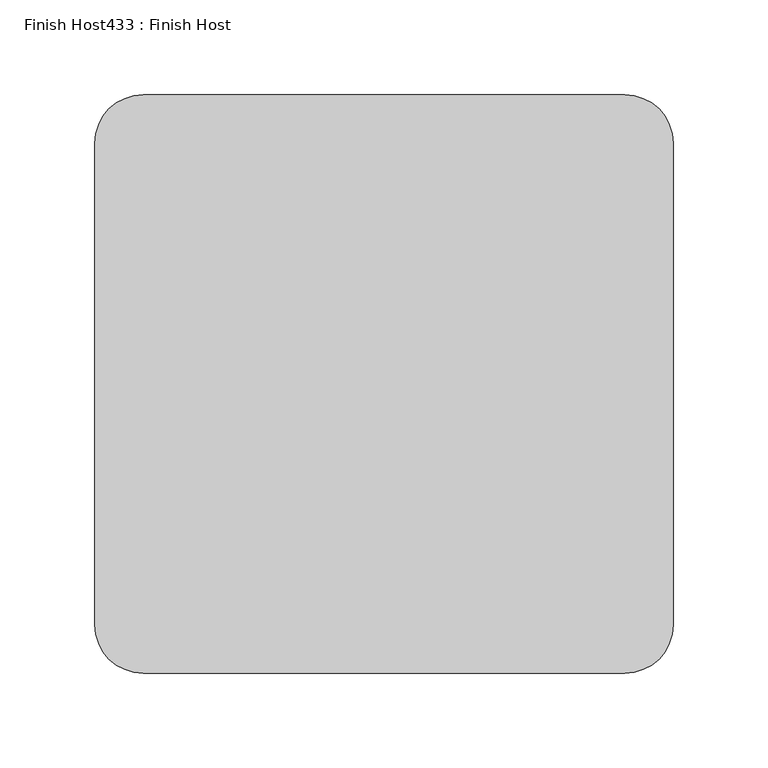
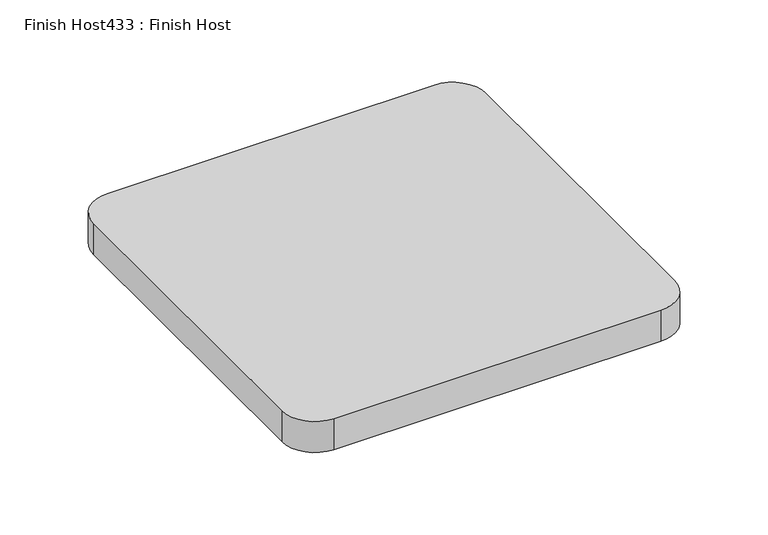
"""IFC4 building model written with IfcOpenShell, lengths in millimetres: proxy geometry, Finish Host433 : Finish Host."""

import ifcopenshell
import ifcopenshell.guid

model = None  # the IFC model being written
_history = None  # IfcOwnerHistory: only IFC2X3 demands one
_inside = {}  # id of a spatial element -> (the spatial element, [elements in it])
_under = {}  # id of a project, library or spatial element -> (it, [spatial elements below it])
_declared = {}  # id of a project -> (the project, [libraries it declares])
_typed = {}  # id of a type object -> (the type object, [elements of that type])
_made_of = {}  # id of a material, layer set ... -> (it, [elements and type objects made of it])


def new_model(schema):
    """Start an empty IFC model of exactly this schema.

    Asked for "IFC4X3", IfcOpenShell would pick the latest addendum, in which some entities
    have other attributes; the version numbers below select the first issue.
    IFC2X3 requires an IfcOwnerHistory on every rooted entity: one is made here for all.
    """
    global model, _history
    if schema == "IFC4X3":
        model = ifcopenshell.file(schema_version=(4, 3, 0, 0))
    else:
        model = ifcopenshell.file(schema=schema)
    _inside.clear()
    _under.clear()
    _declared.clear()
    _typed.clear()
    _made_of.clear()
    _history = None
    if model.schema == "IFC2X3":
        org = make("IfcOrganization", Name="unknown")
        user = make(
            "IfcPersonAndOrganization",
            ThePerson=make("IfcPerson", FamilyName="unknown"),
            TheOrganization=org,
        )
        app = make(
            "IfcApplication",
            ApplicationDeveloper=org,
            Version="unknown",
            ApplicationFullName="unknown",
            ApplicationIdentifier="unknown",
        )
        _history = make(
            "IfcOwnerHistory",
            OwningUser=user,
            OwningApplication=app,
            ChangeAction="ADDED",
            CreationDate=0,
        )
    return model


def make(cls, **values):
    """One entity of the class cls with the attributes given. An attribute that is None is left unset."""
    return model.create_entity(
        cls, **{name: value for name, value in values.items() if value is not None}
    )


def rooted(cls, **values):
    """An entity with a GlobalId (a new one), such as an element, a storey or a relation."""
    return make(cls, GlobalId=ifcopenshell.guid.new(), OwnerHistory=_history, **values)


def si_unit(unit_type, name, prefix=None):
    """IfcSIUnit, for example si_unit("LENGTHUNIT", "METRE", prefix="MILLI")."""
    return make("IfcSIUnit", UnitType=unit_type, Prefix=prefix, Name=name)


def assignment(units):
    """IfcUnitAssignment: the units of a project."""
    return None if units is None else make("IfcUnitAssignment", Units=units)


def point(xyz):
    """IfcCartesianPoint."""
    return None if xyz is None else make("IfcCartesianPoint", Coordinates=xyz)


def direction(xyz):
    """IfcDirection."""
    return None if xyz is None else make("IfcDirection", DirectionRatios=xyz)


def frame(location, z_axis=None, x_axis=None):
    """IfcAxis2Placement3D, a coordinate frame: its origin and axes. An axis left out is left unset."""
    return make(
        "IfcAxis2Placement3D",
        Location=point(location),
        Axis=direction(z_axis),
        RefDirection=direction(x_axis),
    )


def frame_2d(location, x_axis=None):
    """IfcAxis2Placement2D, a coordinate frame in the plane: its origin and x axis."""
    return make(
        "IfcAxis2Placement2D", Location=point(location), RefDirection=direction(x_axis)
    )


def origin():
    """The frame at (0, 0, 0) with its axes left unset."""
    return frame((0.0, 0.0, 0.0))


def origin_with_axes():
    """The frame at (0, 0, 0) with the z axis (0, 0, 1) and the x axis (1, 0, 0) written out."""
    return frame((0.0, 0.0, 0.0), z_axis=(0.0, 0.0, 1.0), x_axis=(1.0, 0.0, 0.0))


def place(relative_to, where):
    """IfcLocalPlacement: puts the frame where relative to a parent placement (None: the world)."""
    return make(
        "IfcLocalPlacement", PlacementRelTo=relative_to, RelativePlacement=where
    )


def context(
    kind, dimensions, precision=None, world=None, true_north=None, identifier=None
):
    """IfcGeometricRepresentationContext, for example the 3D "Model" context."""
    return make(
        "IfcGeometricRepresentationContext",
        ContextIdentifier=identifier,
        ContextType=kind,
        CoordinateSpaceDimension=dimensions,
        Precision=precision,
        WorldCoordinateSystem=world,
        TrueNorth=true_north,
    )


def project(units=None, contexts=None):
    """IfcProject with its units and contexts."""
    return rooted(
        "IfcProject",
        Name="project",
        RepresentationContexts=contexts,
        UnitsInContext=assignment(units),
    )


def spatial(cls, under=None, at=None, **own):
    """A site, building, storey or space (cls), placed at a placement, below another one or the project."""
    s = rooted(cls, ObjectPlacement=at, **own)
    if under is not None:
        _under.setdefault(under.id(), (under, []))[1].append(s)
    return s


def polyline(points):
    """IfcPolyline through the points."""
    return make("IfcPolyline", Points=[point(p) for p in points])


def circle_curve(where, radius):
    """IfcCircle in the frame where."""
    return make("IfcCircle", Position=where, Radius=radius)


def trimmed(basis, trim1, trim2, sense, master):
    """IfcTrimmedCurve: the piece of a basis curve between two trims."""
    return make(
        "IfcTrimmedCurve",
        BasisCurve=basis,
        Trim1=trim1,
        Trim2=trim2,
        SenseAgreement=sense,
        MasterRepresentation=master,
    )


def segment(curve, same_sense, transition):
    """IfcCompositeCurveSegment."""
    return make(
        "IfcCompositeCurveSegment",
        Transition=transition,
        SameSense=same_sense,
        ParentCurve=curve,
    )


def composite_curve(segments, self_intersect=None):
    """IfcCompositeCurve: segments joined end to end."""
    return make("IfcCompositeCurve", Segments=segments, SelfIntersect=self_intersect)


def outline(outer, holes=None, kind="AREA"):
    """IfcArbitraryClosedProfileDef: a profile drawn as a closed curve; with holes, ...WithVoids."""
    if holes is None:
        return make("IfcArbitraryClosedProfileDef", ProfileType=kind, OuterCurve=outer)
    return make(
        "IfcArbitraryProfileDefWithVoids",
        ProfileType=kind,
        OuterCurve=outer,
        InnerCurves=holes,
    )


def extrude(swept, where, along, depth):
    """IfcExtrudedAreaSolid: the profile swept, set in the frame where, extruded along a direction by depth."""
    return make(
        "IfcExtrudedAreaSolid",
        SweptArea=swept,
        Position=where,
        ExtrudedDirection=direction(along),
        Depth=depth,
    )


def shape(context_of_items, identifier, shape_type, items):
    """IfcShapeRepresentation: the items that make up one representation, for example the "Body"."""
    return make(
        "IfcShapeRepresentation",
        ContextOfItems=context_of_items,
        RepresentationIdentifier=identifier,
        RepresentationType=shape_type,
        Items=items,
    )


def source(mapping_origin, context_of_items, identifier, shape_type, items):
    """IfcRepresentationMap: a shape defined once, which mapped items show again and again."""
    return make(
        "IfcRepresentationMap",
        MappingOrigin=mapping_origin,
        MappedRepresentation=shape(context_of_items, identifier, shape_type, items),
    )


def transform(
    local_origin,
    x_axis=None,
    y_axis=None,
    z_axis=None,
    scale=None,
    scale2=None,
    scale3=None,
    uniform=True,
):
    """IfcCartesianTransformationOperator3D, or its non-uniform kind. x_axis, y_axis, z_axis: its Axis1, 2, 3."""
    if uniform:
        return make(
            "IfcCartesianTransformationOperator3D",
            Axis1=direction(x_axis),
            Axis2=direction(y_axis),
            LocalOrigin=point(local_origin),
            Scale=scale,
            Axis3=direction(z_axis),
        )
    return make(
        "IfcCartesianTransformationOperator3DnonUniform",
        Axis1=direction(x_axis),
        Axis2=direction(y_axis),
        LocalOrigin=point(local_origin),
        Scale=scale,
        Axis3=direction(z_axis),
        Scale2=scale2,
        Scale3=scale3,
    )


def mapped(mapping_source, mapping_target):
    """IfcMappedItem: shows the shape of a source again, moved by a transform."""
    return make(
        "IfcMappedItem", MappingSource=mapping_source, MappingTarget=mapping_target
    )


def made_of(thing, what):
    """Note that an element or type object is made of a material, layer set ...; save() writes the relation."""
    if what is not None:
        _made_of.setdefault(what.id(), (what, []))[1].append(thing)
    return thing


def element(
    cls,
    number,
    at=None,
    inside=None,
    cuts=None,
    type_object=None,
    material=None,
    context=None,
    identifier="Body",
    shape_type=None,
    held_by="IfcProductDefinitionShape",
    body=None,
    shapes=None,
    **own,
):
    """One element of the class cls, such as IfcWall. Its Tag is "e" and its number.

    at: its placement. inside: the storey or other place that contains it. cuts: it is an
    opening in that element (IfcRelVoidsElement). A single representation is given by context,
    identifier, shape_type and body (its items); several are given by shapes. held_by: the class
    of the entity that holds the representations. save() writes the other relations.
    """
    e = rooted(cls, Tag="e%d" % number, ObjectPlacement=at, **own)
    if body is not None:
        shapes = [shape(context, identifier, shape_type, body)]
    if shapes is not None:
        e.Representation = make(held_by, Representations=shapes)
    if inside is not None:
        _inside.setdefault(inside.id(), (inside, []))[1].append(e)
    if cuts is not None:
        rooted(
            "IfcRelVoidsElement", RelatingBuildingElement=cuts, RelatedOpeningElement=e
        )
    if type_object is not None:
        _typed.setdefault(type_object.id(), (type_object, []))[1].append(e)
    return made_of(e, material)


def aggregate(whole, parts):
    """IfcRelAggregates: a whole, such as a stair, and the parts it consists of."""
    return rooted("IfcRelAggregates", RelatingObject=whole, RelatedObjects=parts)


def save(model, path):
    """Write the relations noted so far, then the file.

    IfcRelAggregates (storeys below a building ...), IfcRelContainedInSpatialStructure (elements
    in a storey), IfcRelDefinesByType, IfcRelAssociatesMaterial and IfcRelDeclares: one each for
    every whole, place, type object, material and project.
    """
    for whole, parts in _under.values():
        aggregate(whole, parts)
    for where, things in _inside.values():
        rooted(
            "IfcRelContainedInSpatialStructure",
            RelatedElements=things,
            RelatingStructure=where,
        )
    for kind, things in _typed.values():
        rooted("IfcRelDefinesByType", RelatedObjects=things, RelatingType=kind)
    for what, things in _made_of.values():
        rooted("IfcRelAssociatesMaterial", RelatedObjects=things, RelatingMaterial=what)
    for by, libraries in _declared.values():
        rooted("IfcRelDeclares", RelatingContext=by, RelatedDefinitions=libraries)
    model.write(path)


def finish_host433_finish_host_1bc90c5f(model_context):
    return source(origin(), model_context, "Body", "SweptSolid", [
        extrude(outline(composite_curve([segment(polyline([(701.4157184, 4661.2760864), (701.4157184, 4915.2760864)]), True, "CONTINUOUS"), segment(trimmed(circle_curve(frame_2d((726.8157184, 4915.2760864)), 25.4), [point((701.4157184, 4915.2760864))], [point((726.8157184, 4940.6760864))], False, "CARTESIAN"), True, "CONTINUOUS"), segment(polyline([(726.8157184, 4940.6760864), (980.8157184, 4940.6760864)]), True, "CONTINUOUS"), segment(trimmed(circle_curve(frame_2d((980.8157184, 4915.2760864)), 25.4), [point((980.8157184, 4940.6760864))], [point((1006.2157184, 4915.2760864))], False, "CARTESIAN"), True, "CONTINUOUS"), segment(polyline([(1006.2157184, 4915.2760864), (1006.2157184, 4661.2760864)]), True, "CONTINUOUS"), segment(trimmed(circle_curve(frame_2d((980.8157184, 4661.2760864)), 25.4), [point((1006.2157184, 4661.2760864))], [point((980.8157184, 4635.8760864))], False, "CARTESIAN"), True, "CONTINUOUS"), segment(polyline([(980.8157184, 4635.8760864), (726.8157184, 4635.8760864)]), True, "CONTINUOUS"), segment(trimmed(circle_curve(frame_2d((726.8157184, 4661.2760864)), 25.4), [point((726.8157184, 4635.8760864))], [point((701.4157184, 4661.2760864))], False, "CARTESIAN"), True, "CONTINUOUS")], self_intersect=False)), origin_with_axes(), (0.0, 0.0, 1.0), 25.4),
    ])


if __name__ == "__main__":
    model = new_model("IFC4")
    model_context = context("Model", 3, world=origin())
    ifc_project = project(units=[si_unit("LENGTHUNIT", "METRE", prefix="MILLI")], contexts=[model_context])
    site = spatial("IfcSite", under=ifc_project)
    building = spatial("IfcBuilding", under=site)
    placement = place(None, origin())
    finish_host433_finish_host_shape = finish_host433_finish_host_1bc90c5f(model_context)
    element("IfcBuildingElementProxy", 1, Name="Finish Host433 : Finish Host", ObjectType="Finish Host433 : Finish Host", at=placement, inside=building, context=model_context, shape_type="MappedRepresentation", body=[
        mapped(finish_host433_finish_host_shape, transform((0.0, 0.0, 0.0), x_axis=(1.0, 0.0, 0.0), y_axis=(0.0, 1.0, 0.0), z_axis=(0.0, 0.0, 1.0))),
    ])
    save(model, "model.ifc")

# Revit data of these elements
# Type "Finish Host433 : Finish Host"
#   Countertop Material = Paint - Teknion - Accent - Butternut
# Element 1 (IfcBuildingElementProxy, "Finish Host433 : Finish Host")
#   Materials on its faces: "Paint - Teknion - Accent - Butternut"
# Materials
#   "Paint - Teknion - Accent - Butternut": class "Paint", colour RGB 166 137 44, transparency 0, Manufacturer = "Teknion", URL = "http://www.teknion.com/", Description = "Butternut", Cost = 0
